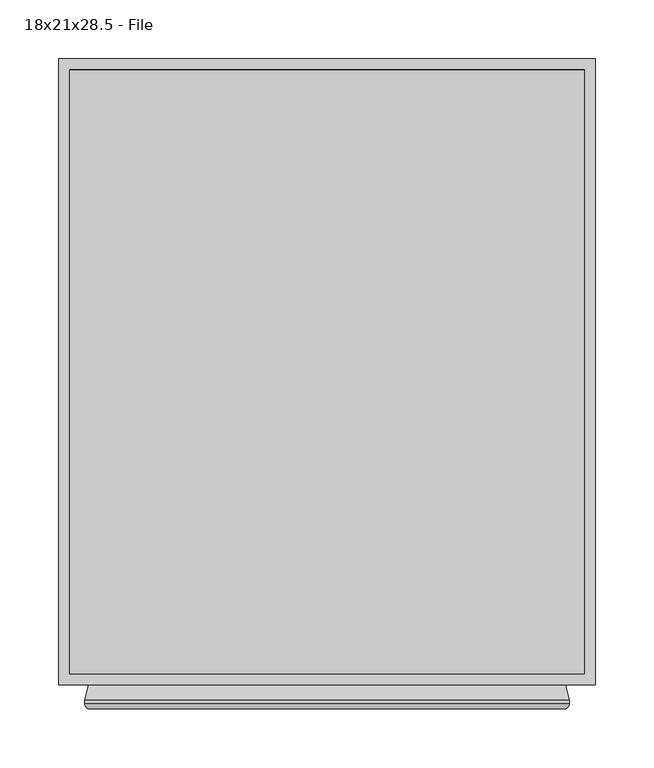
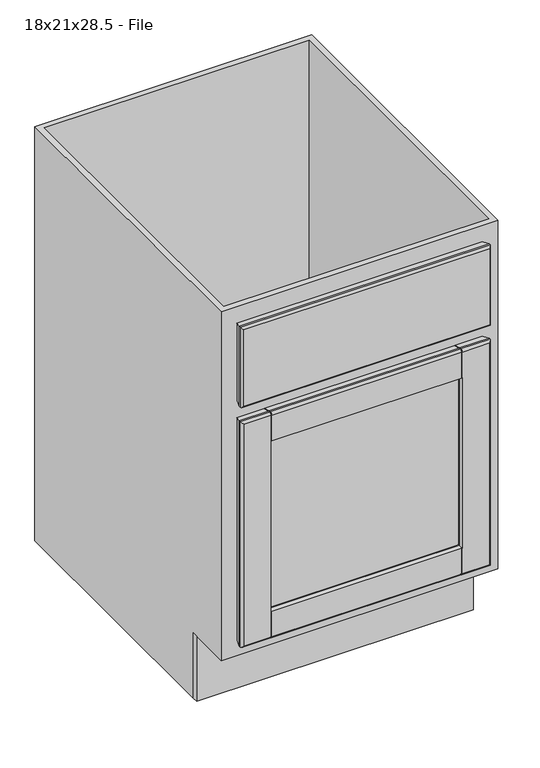
"""IFC4 building model written with IfcOpenShell, lengths in millimetres: furniture geometry, Cabinet-Base-Merillat-Single_Door-Marlin : 18x21x28.5 - File."""

from ifc_helpers import new_model, si_unit, frame, origin, origin_with_axes, place, context, project, spatial, polyline, circle_curve, ellipse_curve, outline, extrude, faceted_brep, source, transform, mapped, element, save
from ifc_brep_helpers import plane_surface, cylinder_surface, advanced_brep


def furniture_18x21x28_5_file_078d9ba0(model_context):
    return source(origin(), model_context, "Body", "SolidModel", [
        advanced_brep(
        [(225.1127049, -625.4496, 533.4), (222.0162124, -629.92, 530.3035075), (222.0162124, -629.92, 142.7964925), (225.1127049, -625.4496, 139.7), (225.1127049, -622.681, 139.7), (225.1127049, -622.681, 533.4), (221.6075049, -609.6, 143.2052), (221.6075049, -609.6, 529.8948), (176.9115422, -609.6, 485.1988372), (176.9115422, -609.6, 187.9011628), (176.5414105, -610.39375, 188.2712945), (174.4602514, -614.85681, 190.3524535), (174.4602514, -614.85681, 482.7475465), (176.5414105, -610.39375, 484.8287055), (175.8600209, -617.0969093, 188.952684), (175.8600209, -617.0969093, 484.147316), (190.1877049, -617.347, 174.625), (190.1877049, -617.347, 498.475), (190.1877049, -622.173, 174.625), (190.1877049, -622.173, 498.475), (175.8600209, -622.4230907, 188.952684), (175.8600209, -622.4230907, 484.147316), (174.4602514, -624.66319, 190.3524535), (174.4602514, -624.66319, 482.7475465), (176.5414105, -629.12625, 188.2712945), (176.9086747, -629.9138508, 187.9040302), (176.9115422, -629.92, 485.1988372), (176.5414105, -629.12625, 484.8287055), (176.9086747, -629.92, 142.7964925), (176.9086747, -625.4496, 139.7), (-184.5408026, -629.92, 142.7964925), (-187.6372951, -625.4496, 139.7), (-139.4730764, -625.4496, 139.7), (-139.4730764, -629.92, 142.7964925), (175.3211747, -625.4496, 139.7), (175.3211747, -629.92, 142.7964925), (-137.8855764, -629.92, 142.7964925), (-137.8855764, -625.4496, 139.7), (176.9086747, -622.681, 139.7), (-187.6372951, -622.681, 139.7), (-139.4730764, -622.681, 139.7), (175.3211747, -622.681, 139.7), (-137.8855764, -622.681, 139.7), (176.9086747, -609.6, 143.2052), (-184.1320951, -609.6, 143.2052), (-139.4730764, -609.6, 143.2052), (175.3211747, -609.6, 143.2052), (-137.8855764, -609.6, 143.2052), (-136.9848416, -614.85681, 190.3524535), (175.3211747, -610.39375, 188.2712945), (175.3211747, -609.6, 187.9011628), (-137.8855764, -609.6, 187.9011628), (-137.8855764, -610.39375, 188.2712945), (-139.0660006, -610.39375, 188.2712945), (-138.384611, -617.0969093, 188.952684), (-152.7122951, -617.347, 174.625), (-152.7122951, -622.173, 174.625), (-138.384611, -622.4230907, 188.952684), (-136.9848416, -624.66319, 190.3524535), (-139.0660006, -629.12625, 188.2712945), (-137.8855764, -629.12625, 188.2712945), (-137.8855764, -629.92, 187.9011628), (175.3211747, -629.92, 187.9011628), (175.3211747, -629.12625, 188.2712945), (-184.5408026, -629.92, 530.3035075), (-187.6372951, -625.4496, 533.4), (-187.6372951, -622.681, 533.4), (-184.1320951, -609.6, 529.8948), (-139.4361323, -609.6, 187.9011628), (-139.4361323, -609.6, 485.1988372), (-139.0660006, -610.39375, 484.8287055), (-136.9848416, -614.85681, 482.7475465), (-138.384611, -617.0969093, 484.147316), (-152.7122951, -617.347, 498.475), (-152.7122951, -622.173, 498.475), (-138.384611, -622.4230907, 484.147316), (-136.9848416, -624.66319, 482.7475465), (-139.0660006, -629.12625, 484.8287055), (-139.4361323, -629.92, 485.1988372), (-139.4361323, -629.92, 187.9011628), (-139.4730764, -629.92, 530.3035075), (-139.4730764, -625.4496, 533.4), (176.9086747, -625.4496, 533.4), (176.9086747, -629.92, 530.3035075), (-137.8855764, -625.4496, 533.4), (-137.8855764, -629.92, 530.3035075), (175.3211747, -629.92, 530.3035075), (175.3211747, -625.4496, 533.4), (-139.4730764, -622.681, 533.4), (176.9086747, -622.681, 533.4), (-137.8855764, -622.681, 533.4), (175.3211747, -622.681, 533.4), (-139.4730764, -609.6, 529.8948), (176.9086747, -609.6, 529.8948), (-137.8855764, -609.6, 529.8948), (175.3211747, -609.6, 529.8948), (-137.8855764, -609.6, 485.1988372), (175.3211747, -609.6, 485.1988372), (-137.8855764, -610.39375, 484.8287055), (175.3211747, -610.39375, 484.8287055), (175.3211747, -629.12625, 484.8287055), (175.3211747, -629.92, 485.1988372), (-137.8855764, -629.92, 485.1988372), (-137.8855764, -629.12625, 484.8287055), (-137.8855764, -610.39375, 529.2857412), (-137.8855764, -622.7855037, 532.60625), (-137.8855764, -625.4496, 532.60625), (-137.8855764, -629.12625, 530.1526052), (-139.4730764, -629.12625, 484.8287055), (-139.4730764, -629.12625, 530.1526052), (-139.4730764, -625.4496, 532.60625), (-139.4730764, -622.7855037, 532.60625), (-139.4730764, -610.39375, 529.2857412), (-139.4730764, -610.39375, 484.8287055), (176.9086747, -610.39375, 484.8287055), (176.9086747, -610.39375, 529.2857412), (176.9086747, -622.7855037, 532.60625), (176.9086747, -625.4496, 532.60625), (176.9086747, -629.12625, 530.1526052), (176.9086747, -629.12625, 484.8287055), (175.3211747, -629.12625, 530.1526052), (175.3211747, -625.4496, 532.60625), (175.3211747, -622.7855037, 532.60625), (175.3211747, -610.39375, 529.2857412), (176.9086747, -629.12625, 188.2712945), (176.9086747, -629.12625, 142.9473948), (176.9086747, -625.4496, 140.49375), (176.9086747, -622.7855037, 140.49375), (176.9086747, -610.39375, 143.8142588), (176.9086747, -610.39375, 188.2712945), (175.3211747, -610.39375, 143.8142588), (175.3211747, -622.7855037, 140.49375), (175.3211747, -625.4496, 140.49375), (175.3211747, -629.12625, 142.9473948), (-137.8855764, -629.12625, 142.9473948), (-137.8855764, -625.4496, 140.49375), (-137.8855764, -622.7855037, 140.49375), (-137.8855764, -610.39375, 143.8142588), (-139.4730764, -629.12625, 188.2712945), (-139.4730764, -610.39375, 188.2712945), (-139.4730764, -610.39375, 143.8142588), (-139.4730764, -622.7855037, 140.49375), (-139.4730764, -625.4496, 140.49375), (-139.4730764, -629.12625, 142.9473948)],
        [
            (0, 1, ellipse_curve(frame((220.3375049, -625.4496, 528.6248), z_axis=(0.7071067811865475, 0.0, -0.7071067811865475), x_axis=(0.7071067811865474, 0.0, 0.7071067811865476)), 6.7531526, 4.7752)),
            (1, 2),
            (2, 3, ellipse_curve(frame((220.3375049, -625.4496, 144.4752), z_axis=(0.7071067811865475, 0.0, 0.7071067811865475), x_axis=(-0.7071067811865474, 0.0, 0.7071067811865476)), 6.7531526, 4.7752)),
            (3, 0),
            (3, 4),
            (4, 5),
            (5, 0),
            (4, 6),
            (6, 7),
            (7, 5),
            (8, 9),
            (9, 10),
            (10, 11),
            (11, 12),
            (12, 13),
            (13, 8),
            (11, 14, ellipse_curve(frame((175.8875049, -615.5223492, 188.9252), z_axis=(0.7071067811865475, 0.0, 0.7071067811865475), x_axis=(-0.7071067811865474, 0.0, 0.7071067811865476)), 2.2271035, 1.5748)),
            (14, 15),
            (15, 12, ellipse_curve(frame((175.8875049, -615.5223492, 484.1748), z_axis=(0.7071067811865475, 0.0, -0.7071067811865475), x_axis=(0.7071067811865474, 0.0, 0.7071067811865476)), 2.2271035, 1.5748)),
            (14, 16),
            (16, 17),
            (17, 15),
            (16, 18),
            (18, 19),
            (19, 17),
            (18, 20),
            (20, 21),
            (21, 19),
            (20, 22, ellipse_curve(frame((175.8875049, -623.9976508, 188.9252), z_axis=(0.7071067811865475, 0.0, 0.7071067811865475), x_axis=(-0.7071067811865474, 0.0, 0.7071067811865476)), 2.2271035, 1.5748)),
            (22, 23),
            (23, 21, ellipse_curve(frame((175.8875049, -623.9976508, 484.1748), z_axis=(0.7071067811865475, 0.0, -0.7071067811865475), x_axis=(0.7071067811865474, 0.0, 0.7071067811865476)), 2.2271035, 1.5748)),
            (22, 24),
            (24, 25),
            (25, 26),
            (26, 27),
            (27, 23),
            (2, 28),
            (28, 29, circle_curve(frame((176.9086747, -625.4496, 144.4752), z_axis=(1.0, 0.0, 0.0), x_axis=(0.0, 1.0, 0.0)), 4.7752)),
            (29, 3),
            (30, 31, ellipse_curve(frame((-182.8620951, -625.4496, 144.4752), z_axis=(0.7071067811865475, 0.0, -0.7071067811865475), x_axis=(0.7071067811865476, 0.0, 0.7071067811865474)), 6.7531526, 4.7752)),
            (31, 32),
            (32, 33, circle_curve(frame((-139.4730764, -625.4496, 144.4752), z_axis=(-1.0, 0.0, 0.0), x_axis=(0.0, 1.0, 0.0)), 4.7752)),
            (33, 30),
            (34, 35, circle_curve(frame((175.3211747, -625.4496, 144.4752), z_axis=(-1.0, 0.0, 0.0), x_axis=(0.0, 1.0, 0.0)), 4.7752)),
            (35, 36),
            (36, 37, circle_curve(frame((-137.8855764, -625.4496, 144.4752), z_axis=(1.0, 0.0, 0.0), x_axis=(0.0, 1.0, 0.0)), 4.7752)),
            (37, 34),
            (29, 38),
            (38, 4),
            (31, 39),
            (39, 40),
            (40, 32),
            (41, 34),
            (37, 42),
            (42, 41),
            (38, 43),
            (43, 6),
            (39, 44),
            (44, 45),
            (45, 40),
            (46, 41),
            (42, 47),
            (47, 46),
            (48, 11),
            (10, 49),
            (49, 50),
            (50, 51),
            (51, 52),
            (52, 53),
            (53, 48),
            (48, 54, ellipse_curve(frame((-138.4120951, -615.5223492, 188.9252), z_axis=(0.7071067811865475, 0.0, -0.7071067811865475), x_axis=(0.7071067811865476, 0.0, 0.7071067811865474)), 2.2271035, 1.5748)),
            (54, 14),
            (54, 55),
            (55, 16),
            (55, 56),
            (56, 18),
            (56, 57),
            (57, 20),
            (57, 58, ellipse_curve(frame((-138.4120951, -623.9976508, 188.9252), z_axis=(0.7071067811865475, 0.0, -0.7071067811865475), x_axis=(0.7071067811865476, 0.0, 0.7071067811865474)), 2.2271035, 1.5748)),
            (58, 22),
            (58, 59),
            (59, 60),
            (60, 61),
            (61, 62),
            (62, 63),
            (63, 24),
            (30, 64),
            (64, 65, ellipse_curve(frame((-182.8620951, -625.4496, 528.6248), z_axis=(-0.7071067811865475, 0.0, -0.7071067811865475), x_axis=(0.7071067811865474, 0.0, -0.7071067811865476)), 6.7531526, 4.7752)),
            (65, 31),
            (65, 66),
            (66, 39),
            (66, 67),
            (67, 44),
            (68, 69),
            (69, 70),
            (70, 71),
            (71, 48),
            (53, 68),
            (71, 72, ellipse_curve(frame((-138.4120951, -615.5223492, 484.1748), z_axis=(-0.7071067811865475, 0.0, -0.7071067811865475), x_axis=(0.7071067811865474, 0.0, -0.7071067811865476)), 2.2271035, 1.5748)),
            (72, 54),
            (72, 73),
            (73, 55),
            (73, 74),
            (74, 56),
            (74, 75),
            (75, 57),
            (75, 76, ellipse_curve(frame((-138.4120951, -623.9976508, 484.1748), z_axis=(-0.7071067811865475, 0.0, -0.7071067811865475), x_axis=(0.7071067811865474, 0.0, -0.7071067811865476)), 2.2271035, 1.5748)),
            (76, 58),
            (76, 77),
            (77, 78),
            (78, 79),
            (79, 59),
            (64, 80),
            (80, 81, circle_curve(frame((-139.4730764, -625.4496, 528.6248), z_axis=(-1.0, 0.0, 0.0), x_axis=(0.0, 1.0, 0.0)), 4.7752)),
            (81, 65),
            (0, 82),
            (82, 83, circle_curve(frame((176.9086747, -625.4496, 528.6248), z_axis=(1.0, 0.0, 0.0), x_axis=(0.0, 1.0, 0.0)), 4.7752)),
            (83, 1),
            (84, 85, circle_curve(frame((-137.8855764, -625.4496, 528.6248), z_axis=(1.0, 0.0, 0.0), x_axis=(0.0, 1.0, 0.0)), 4.7752)),
            (85, 86),
            (86, 87, circle_curve(frame((175.3211747, -625.4496, 528.6248), z_axis=(-1.0, 0.0, 0.0), x_axis=(0.0, 1.0, 0.0)), 4.7752)),
            (87, 84),
            (81, 88),
            (88, 66),
            (5, 89),
            (89, 82),
            (90, 84),
            (87, 91),
            (91, 90),
            (88, 92),
            (92, 67),
            (7, 93),
            (93, 89),
            (94, 90),
            (91, 95),
            (95, 94),
            (43, 9),
            (8, 93),
            (92, 69),
            (68, 45),
            (96, 94),
            (95, 97),
            (97, 96),
            (50, 46),
            (47, 51),
            (12, 71),
            (70, 98),
            (98, 96),
            (97, 99),
            (99, 13),
            (15, 72),
            (17, 73),
            (19, 74),
            (21, 75),
            (23, 76),
            (27, 100),
            (100, 101),
            (101, 102),
            (102, 103),
            (103, 77),
            (83, 26),
            (25, 28),
            (33, 79),
            (78, 80),
            (85, 102),
            (101, 86),
            (35, 62),
            (61, 36),
            (98, 104),
            (104, 105),
            (105, 106),
            (106, 107, circle_curve(frame((-137.8855764, -625.4496, 528.6248), z_axis=(1.0, 0.0, 0.0), x_axis=(0.0, 0.0, 1.0)), 3.98145)),
            (107, 103),
            (78, 108),
            (108, 109),
            (109, 110, circle_curve(frame((-139.4730764, -625.4496, 528.6248), z_axis=(-1.0, 0.0, 0.0), x_axis=(0.0, 0.0, 1.0)), 3.98145)),
            (110, 111),
            (111, 112),
            (112, 113),
            (113, 69),
            (77, 108),
            (107, 109),
            (106, 110),
            (105, 111),
            (104, 112),
            (70, 113),
            (8, 114),
            (114, 115),
            (115, 116),
            (116, 117),
            (117, 118, circle_curve(frame((176.9086747, -625.4496, 528.6248), z_axis=(1.0, 0.0, 0.0), x_axis=(0.0, 0.0, 1.0)), 3.98145)),
            (118, 119),
            (119, 26),
            (100, 120),
            (120, 121, circle_curve(frame((175.3211747, -625.4496, 528.6248), z_axis=(-1.0, 0.0, 0.0), x_axis=(0.0, 0.0, 1.0)), 3.98145)),
            (121, 122),
            (122, 123),
            (123, 99),
            (119, 27),
            (118, 120),
            (117, 121),
            (116, 122),
            (115, 123),
            (114, 13),
            (25, 124),
            (124, 125),
            (125, 126, circle_curve(frame((176.9086747, -625.4496, 144.4752), z_axis=(1.0, 0.0, 0.0), x_axis=(0.0, 0.0, 1.0)), 3.98145)),
            (126, 127),
            (127, 128),
            (128, 129),
            (129, 9),
            (49, 130),
            (130, 131),
            (131, 132),
            (132, 133, circle_curve(frame((175.3211747, -625.4496, 144.4752), z_axis=(-1.0, 0.0, 0.0), x_axis=(0.0, 0.0, 1.0)), 3.98145)),
            (133, 63),
            (129, 10),
            (128, 130),
            (127, 131),
            (126, 132),
            (125, 133),
            (124, 24),
            (60, 134),
            (134, 135, circle_curve(frame((-137.8855764, -625.4496, 144.4752), z_axis=(1.0, 0.0, 0.0), x_axis=(0.0, 0.0, 1.0)), 3.98145)),
            (135, 136),
            (136, 137),
            (137, 52),
            (138, 79),
            (68, 139),
            (139, 140),
            (140, 141),
            (141, 142),
            (142, 143, circle_curve(frame((-139.4730764, -625.4496, 144.4752), z_axis=(-1.0, 0.0, 0.0), x_axis=(0.0, 0.0, 1.0)), 3.98145)),
            (143, 138),
            (138, 59),
            (53, 139),
            (137, 140),
            (136, 141),
            (135, 142),
            (134, 143),
        ],
        [
            cylinder_surface(frame((220.3375049, -625.4496, 533.4), z_axis=(0.0, 0.0, 1.0), x_axis=(0.0, 1.0, 0.0)), 4.7752),
            plane_surface(frame((225.1127049, -625.4496, 533.4), z_axis=(1.0, 0.0, 0.0), x_axis=(0.0, 0.0, -1.0))),
            plane_surface(frame((225.1127049, -622.681, 533.4), z_axis=(0.9659229350723619, 0.25882983502910506, 0.0), x_axis=(0.0, 0.0, -1.0))),
            plane_surface(frame((176.9115422, -609.6, 485.1988372), z_axis=(-0.9063077870366099, 0.4226182617407856, 0.0), x_axis=(0.0, 0.0, -1.0))),
            cylinder_surface(frame((175.8875049, -615.5223492, 533.4), z_axis=(0.0, 0.0, 1.0000000000000002), x_axis=(-0.01745240643729364, -0.9998476951563912, 0.0)), 1.5748),
            plane_surface(frame((175.8600209, -617.0969093, 484.147316), z_axis=(-0.017452406437322144, -0.9998476951563906, 0.0), x_axis=(0.0, 0.0, -1.0))),
            plane_surface(frame((190.1877049, -617.347, 498.475), z_axis=(-1.0, 0.0, 0.0), x_axis=(0.0, 0.0, -1.0))),
            plane_surface(frame((190.1877049, -622.173, 498.475), z_axis=(-0.01745240643727848, 0.9998476951563914, 0.0), x_axis=(0.0, 0.0, -1.0))),
            cylinder_surface(frame((175.8875049, -623.9976508, 533.4), z_axis=(0.0, 0.0, 1.0000000000000002), x_axis=(-0.9063077870367326, -0.42261826174052236, 0.0)), 1.5748),
            plane_surface(frame((174.4602514, -624.66319, 482.7475465), z_axis=(-0.9063077870366333, -0.4226182617407352, 0.0), x_axis=(0.0, 0.0, -1.0))),
            cylinder_surface(frame((225.1127049, -625.4496, 144.4752), z_axis=(1.0, 0.0, 0.0), x_axis=(0.0, 1.0, 0.0)), 4.7752),
            plane_surface(frame((225.1127049, -625.4496, 139.7), z_axis=(0.0, 0.0, -1.0), x_axis=(-1.0, 0.0, 0.0))),
            plane_surface(frame((225.1127049, -622.681, 139.7), z_axis=(0.0, 0.25882983502910506, -0.9659229350723619), x_axis=(-1.0, 0.0, 0.0))),
            plane_surface(frame((176.9115422, -609.6, 187.9011628), z_axis=(0.0, 0.4226182617407856, 0.9063077870366099), x_axis=(-1.0, 0.0, 0.0))),
            cylinder_surface(frame((225.1127049, -615.5223492, 188.9252), z_axis=(1.0000000000000002, 0.0, 0.0), x_axis=(0.0, -0.9998476951563912, 0.01745240643729364)), 1.5748),
            plane_surface(frame((175.8600209, -617.0969093, 188.952684), z_axis=(0.0, -0.9998476951563906, 0.017452406437322144), x_axis=(-1.0, 0.0, 0.0))),
            plane_surface(frame((190.1877049, -617.347, 174.625), z_axis=(0.0, 0.0, 1.0), x_axis=(-1.0, 0.0, 0.0))),
            plane_surface(frame((190.1877049, -622.173, 174.625), z_axis=(0.0, 0.9998476951563914, 0.01745240643727848), x_axis=(-1.0, 0.0, 0.0))),
            cylinder_surface(frame((225.1127049, -623.9976508, 188.9252), z_axis=(1.0000000000000002, 0.0, 0.0), x_axis=(0.0, -0.42261826174052236, 0.9063077870367326)), 1.5748),
            plane_surface(frame((174.4602514, -624.66319, 190.3524535), z_axis=(0.0, -0.4226182617407352, 0.9063077870366333), x_axis=(-1.0, 0.0, 0.0))),
            cylinder_surface(frame((-182.8620951, -625.4496, 139.7), z_axis=(0.0, 0.0, -1.0), x_axis=(0.0, 1.0, 0.0)), 4.7752),
            plane_surface(frame((-187.6372951, -625.4496, 139.7), z_axis=(-1.0, 0.0, 0.0), x_axis=(0.0, 0.0, 1.0))),
            plane_surface(frame((-187.6372951, -622.681, 139.7), z_axis=(-0.9659229350723619, 0.25882983502910506, 0.0), x_axis=(0.0, 0.0, 1.0))),
            plane_surface(frame((-139.4361323, -609.6, 187.9011628), z_axis=(0.9063077870366099, 0.4226182617407856, 0.0), x_axis=(0.0, 0.0, 1.0))),
            cylinder_surface(frame((-138.4120951, -615.5223492, 139.7), z_axis=(0.0, 0.0, -1.0000000000000002), x_axis=(0.01745240643729364, -0.9998476951563912, 0.0)), 1.5748),
            plane_surface(frame((-138.384611, -617.0969093, 188.952684), z_axis=(0.017452406437322144, -0.9998476951563906, 0.0), x_axis=(0.0, 0.0, 1.0))),
            plane_surface(frame((-152.7122951, -617.347, 174.625), z_axis=(1.0, 0.0, 0.0), x_axis=(0.0, 0.0, 1.0))),
            plane_surface(frame((-152.7122951, -622.173, 174.625), z_axis=(0.01745240643727848, 0.9998476951563914, 0.0), x_axis=(0.0, 0.0, 1.0))),
            cylinder_surface(frame((-138.4120951, -623.9976508, 139.7), z_axis=(0.0, 0.0, -1.0000000000000002), x_axis=(0.9063077870367326, -0.42261826174052236, 0.0)), 1.5748),
            plane_surface(frame((-136.9848416, -624.66319, 190.3524535), z_axis=(0.9063077870366333, -0.4226182617407352, 0.0), x_axis=(0.0, 0.0, 1.0))),
            cylinder_surface(frame((-187.6372951, -625.4496, 528.6248), z_axis=(-1.0, 0.0, 0.0), x_axis=(0.0, 1.0, 0.0)), 4.7752),
            plane_surface(frame((-187.6372951, -625.4496, 533.4), z_axis=(0.0, 0.0, 1.0), x_axis=(1.0, 0.0, 0.0))),
            plane_surface(frame((-187.6372951, -622.681, 533.4), z_axis=(0.0, 0.25882983502910506, 0.9659229350723619), x_axis=(1.0, 0.0, 0.0))),
            plane_surface(frame((-184.1320951, -609.6, 529.8948), z_axis=(0.0, 1.0, 0.0), x_axis=(1.0, 0.0, 0.0))),
            plane_surface(frame((-139.4361323, -609.6, 485.1988372), z_axis=(0.0, 0.4226182617407856, -0.9063077870366099), x_axis=(1.0, 0.0, 0.0))),
            cylinder_surface(frame((-187.6372951, -615.5223492, 484.1748), z_axis=(-1.0000000000000002, 0.0, 0.0), x_axis=(0.0, -0.9998476951563912, -0.01745240643729364)), 1.5748),
            plane_surface(frame((-138.384611, -617.0969093, 484.147316), z_axis=(0.0, -0.9998476951563906, -0.017452406437322144), x_axis=(1.0, 0.0, 0.0))),
            plane_surface(frame((-152.7122951, -617.347, 498.475), z_axis=(0.0, 0.0, -1.0), x_axis=(1.0, 0.0, 0.0))),
            plane_surface(frame((-152.7122951, -622.173, 498.475), z_axis=(0.0, 0.9998476951563914, -0.01745240643727848), x_axis=(1.0, 0.0, 0.0))),
            cylinder_surface(frame((-187.6372951, -623.9976508, 484.1748), z_axis=(-1.0000000000000002, 0.0, 0.0), x_axis=(0.0, -0.42261826174052236, -0.9063077870367326)), 1.5748),
            plane_surface(frame((-136.9848416, -624.66319, 482.7475465), z_axis=(0.0, -0.4226182617407352, -0.9063077870366333), x_axis=(1.0, 0.0, 0.0))),
            plane_surface(frame((-139.4361323, -629.92, 485.1988372), z_axis=(0.0, -1.0, 0.0), x_axis=(1.0, 0.0, 0.0))),
            plane_surface(frame((-137.8855764, -629.92, 485.1988372), z_axis=(-1.0000000000000002, 0.0, 0.0), x_axis=(0.0, 0.9063077870366303, -0.4226182617407418))),
            plane_surface(frame((-139.4730764, -629.92, 485.1988372), z_axis=(1.0000000000000002, 0.0, 0.0), x_axis=(0.0, -0.9063077870366303, 0.4226182617407418))),
            plane_surface(frame((-137.8855764, -629.92, 485.1988372), z_axis=(0.0, 0.4226182617407418, 0.9063077870366303), x_axis=(-1.0, 0.0, 0.0))),
            plane_surface(frame((-137.8855764, -629.12625, 484.8287055), z_axis=(0.0, -1.0, 0.0), x_axis=(-1.0, 0.0, 0.0))),
            cylinder_surface(frame((-139.4730764, -625.4496, 528.6248), z_axis=(-1.0, 0.0, 0.0), x_axis=(0.0, 0.0, 1.0)), 3.98145),
            plane_surface(frame((-137.8855764, -625.4496, 532.60625), z_axis=(0.0, 0.0, 1.0), x_axis=(-1.0, 0.0, 0.0))),
            plane_surface(frame((-137.8855764, -622.7855037, 532.60625), z_axis=(0.0, 0.25882983502916795, 0.9659229350723451), x_axis=(-1.0, 0.0, 0.0))),
            plane_surface(frame((-137.8855764, -610.39375, 529.2857412), z_axis=(0.0, 1.0, 0.0), x_axis=(-1.0, 0.0, 0.0))),
            plane_surface(frame((-137.8855764, -610.39375, 484.8287055), z_axis=(0.0, -0.4226182617407951, 0.9063077870366054), x_axis=(-1.0, 0.0, 0.0))),
            plane_surface(frame((176.9086747, -629.92, 485.1988372), z_axis=(-1.0, 0.0, 0.0), x_axis=(0.0, 0.9063077870366284, -0.42261826174074574))),
            plane_surface(frame((175.3211747, -629.92, 485.1988372), z_axis=(1.0, 0.0, 0.0), x_axis=(0.0, -0.9063077870366284, 0.42261826174074574))),
            plane_surface(frame((176.9086747, -629.92, 485.1988372), z_axis=(0.0, 0.42261826174074574, 0.9063077870366284), x_axis=(-1.0, 0.0, 0.0))),
            plane_surface(frame((176.9086747, -629.12625, 484.8287055), z_axis=(0.0, -1.0, 0.0), x_axis=(-1.0, 0.0, 0.0))),
            cylinder_surface(frame((175.3211747, -625.4496, 528.6248), z_axis=(-1.0, 0.0, 0.0), x_axis=(0.0, 0.0, 1.0)), 3.98145),
            plane_surface(frame((176.9086747, -625.4496, 532.60625), z_axis=(0.0, 0.0, 1.0), x_axis=(-1.0, 0.0, 0.0))),
            plane_surface(frame((176.9086747, -622.7855037, 532.60625), z_axis=(0.0, 0.25882983502917023, 0.9659229350723445), x_axis=(-1.0, 0.0, 0.0))),
            plane_surface(frame((176.9086747, -610.39375, 529.2857412), z_axis=(0.0, 1.0, 0.0), x_axis=(-1.0, 0.0, 0.0))),
            plane_surface(frame((176.9086747, -610.39375, 484.8287055), z_axis=(0.0, -0.4226182617408056, 0.9063077870366005), x_axis=(-1.0, 0.0, 0.0))),
            plane_surface(frame((176.9086747, -625.4496, 149.2504), z_axis=(-1.0, 0.0, 0.0), x_axis=(0.0, -1.0, 0.0))),
            plane_surface(frame((175.3211747, -625.4496, 149.2504), z_axis=(1.0, 0.0, 0.0), x_axis=(0.0, 1.0, 0.0))),
            plane_surface(frame((176.9086747, -609.6, 187.9011628), z_axis=(0.0, -0.4226182617407918, -0.906307787036607), x_axis=(-1.0, 0.0, 0.0))),
            plane_surface(frame((176.9086747, -610.39375, 188.2712945), z_axis=(0.0, 1.0, 0.0), x_axis=(-1.0, 0.0, 0.0))),
            plane_surface(frame((176.9086747, -610.39375, 143.8142588), z_axis=(0.0, 0.25882983502943885, -0.9659229350722724), x_axis=(-1.0, 0.0, 0.0))),
            plane_surface(frame((176.9086747, -622.7855037, 140.49375), z_axis=(0.0, 0.0, -1.0), x_axis=(-1.0, 0.0, 0.0))),
            cylinder_surface(frame((175.3211747, -625.4496, 144.4752), z_axis=(-1.0, 0.0, 0.0), x_axis=(0.0, 0.0, 1.0)), 3.98145),
            plane_surface(frame((176.9086747, -629.12625, 142.9473948), z_axis=(0.0, -1.0, 0.0), x_axis=(-1.0, 0.0, 0.0))),
            plane_surface(frame((176.9086747, -629.12625, 188.2712945), z_axis=(0.0, 0.42261826174073464, -0.9063077870366336), x_axis=(-1.0, 0.0, 0.0))),
            plane_surface(frame((-137.8855764, -629.12625, 188.2712945), z_axis=(-1.0, 0.0, 0.0), x_axis=(0.0, -0.9063077870366311, -0.4226182617407399))),
            plane_surface(frame((-139.4730764, -629.12625, 188.2712945), z_axis=(1.0, 0.0, 0.0), x_axis=(0.0, 0.9063077870366311, 0.4226182617407399))),
            plane_surface(frame((-137.8855764, -629.12625, 188.2712945), z_axis=(0.0, 0.4226182617407399, -0.9063077870366311), x_axis=(-1.0, 0.0, 0.0))),
            plane_surface(frame((-137.8855764, -609.6, 187.9011628), z_axis=(0.0, -0.42261826174079353, -0.9063077870366061), x_axis=(-1.0, 0.0, 0.0))),
            plane_surface(frame((-137.8855764, -610.39375, 188.2712945), z_axis=(0.0, 1.0, 0.0), x_axis=(-1.0, 0.0, 0.0))),
            plane_surface(frame((-137.8855764, -610.39375, 143.8142588), z_axis=(0.0, 0.2588298350294384, -0.9659229350722726), x_axis=(-1.0, 0.0, 0.0))),
            plane_surface(frame((-137.8855764, -622.7855037, 140.49375), z_axis=(0.0, 0.0, -1.0), x_axis=(-1.0, 0.0, 0.0))),
            cylinder_surface(frame((-139.4730764, -625.4496, 144.4752), z_axis=(-1.0, 0.0, 0.0), x_axis=(0.0, 0.0, 1.0)), 3.98145),
            plane_surface(frame((-137.8855764, -629.12625, 142.9473948), z_axis=(0.0, -1.0, 0.0), x_axis=(-1.0, 0.0, 0.0))),
        ],
        [
            (0, [[1, 2, 3, 4]]),
            (1, [[-4, 5, 6, 7]]),
            (2, [[-6, 8, 9, 10]]),
            (3, [[11, 12, 13, 14, 15, 16]]),
            (4, [[-14, 17, 18, 19]]),
            (5, [[-18, 20, 21, 22]]),
            (6, [[-21, 23, 24, 25]]),
            (7, [[-24, 26, 27, 28]]),
            (8, [[-27, 29, 30, 31]]),
            (9, [[-30, 32, 33, 34, 35, 36]]),
            (10, [[-3, 37, 38, 39]]),
            (10, [[40, 41, 42, 43]]),
            (10, [[44, 45, 46, 47]]),
            (11, [[-5, -39, 48, 49]]),
            (11, [[50, 51, 52, -41]]),
            (11, [[53, -47, 54, 55]]),
            (12, [[-8, -49, 56, 57]]),
            (12, [[58, 59, 60, -51]]),
            (12, [[61, -55, 62, 63]]),
            (13, [[64, -13, 65, 66, 67, 68, 69, 70]]),
            (14, [[-17, -64, 71, 72]]),
            (15, [[-20, -72, 73, 74]]),
            (16, [[-23, -74, 75, 76]]),
            (17, [[-26, -76, 77, 78]]),
            (18, [[-29, -78, 79, 80]]),
            (19, [[-80, 81, 82, 83, 84, 85, 86, -32]]),
            (20, [[-40, 87, 88, 89]]),
            (21, [[-50, -89, 90, 91]]),
            (22, [[-58, -91, 92, 93]]),
            (23, [[94, 95, 96, 97, -70, 98]]),
            (24, [[-71, -97, 99, 100]]),
            (25, [[-73, -100, 101, 102]]),
            (26, [[-75, -102, 103, 104]]),
            (27, [[-77, -104, 105, 106]]),
            (28, [[-79, -106, 107, 108]]),
            (29, [[-108, 109, 110, 111, 112, -81]]),
            (30, [[-88, 113, 114, 115]]),
            (30, [[-1, 116, 117, 118]]),
            (30, [[119, 120, 121, 122]]),
            (31, [[-90, -115, 123, 124]]),
            (31, [[-7, 125, 126, -116]]),
            (31, [[127, -122, 128, 129]]),
            (32, [[-92, -124, 130, 131]]),
            (32, [[-10, 132, 133, -125]]),
            (32, [[134, -129, 135, 136]]),
            (33, [[-9, -57, 137, -11, 138, -132]]),
            (33, [[-93, -131, 139, -94, 140, -59]]),
            (33, [[141, -136, 142, 143]]),
            (33, [[144, -63, 145, -67]]),
            (34, [[146, -96, 147, 148, -143, 149, 150, -15]]),
            (35, [[-19, 151, -99, -146]]),
            (36, [[-22, 152, -101, -151]]),
            (37, [[-25, 153, -103, -152]]),
            (38, [[-28, 154, -105, -153]]),
            (39, [[-31, 155, -107, -154]]),
            (40, [[-155, -36, 156, 157, 158, 159, 160, -109]]),
            (41, [[-2, -118, 161, -34, 162, -37]]),
            (41, [[-87, -43, 163, -111, 164, -113]]),
            (41, [[165, -158, 166, -120]]),
            (41, [[167, -84, 168, -45]]),
            (42, [[169, 170, 171, 172, 173, -159, -165, -119, -127, -134, -141, -148]]),
            (43, [[174, 175, 176, 177, 178, 179, 180, -139, -130, -123, -114, -164]]),
            (44, [[-174, -110, 181]]),
            (45, [[-173, 182, -175, -181, -160]]),
            (46, [[-172, 183, -176, -182]]),
            (47, [[-171, 184, -177, -183]]),
            (48, [[-170, 185, -178, -184]]),
            (49, [[-169, -147, 186, -179, -185]]),
            (50, [[-180, -186, -95]]),
            (51, [[187, 188, 189, 190, 191, 192, 193, -161, -117, -126, -133, -138]]),
            (52, [[194, 195, 196, 197, 198, -149, -142, -135, -128, -121, -166, -157]]),
            (53, [[-193, 199, -35]]),
            (54, [[-192, 200, -194, -156, -199]]),
            (55, [[-191, 201, -195, -200]]),
            (56, [[-190, 202, -196, -201]]),
            (57, [[-189, 203, -197, -202]]),
            (58, [[-188, 204, -150, -198, -203]]),
            (59, [[-187, -16, -204]]),
            (60, [[205, 206, 207, 208, 209, 210, 211, -137, -56, -48, -38, -162]]),
            (61, [[212, 213, 214, 215, 216, -85, -167, -44, -53, -61, -144, -66]]),
            (62, [[-211, 217, -12]]),
            (63, [[-210, 218, -212, -65, -217]]),
            (64, [[-209, 219, -213, -218]]),
            (65, [[-208, 220, -214, -219]]),
            (66, [[-207, 221, -215, -220]]),
            (67, [[-206, 222, -86, -216, -221]]),
            (68, [[-205, -33, -222]]),
            (69, [[223, 224, 225, 226, 227, -68, -145, -62, -54, -46, -168, -83]]),
            (70, [[228, -163, -42, -52, -60, -140, 229, 230, 231, 232, 233, 234]]),
            (71, [[-228, 235, -112]]),
            (72, [[-229, -98, 236]]),
            (73, [[-227, 237, -230, -236, -69]]),
            (74, [[-226, 238, -231, -237]]),
            (75, [[-225, 239, -232, -238]]),
            (76, [[-224, 240, -233, -239]]),
            (77, [[-223, -82, -235, -234, -240]]),
        ],
    ),
        extrude(outline(polyline([(-152.7122951, -622.173), (-152.7122951, -617.347), (190.1877049, -617.347), (190.1877049, -622.173), (-152.7122951, -622.173)])), frame((0.0, 0.0, 174.625), z_axis=(0.0, 0.0, 1.0), x_axis=(1.0, 0.0, 0.0)), (0.0, 0.0, 1.0), 323.85),
        advanced_brep(
        [(-184.5408026, -629.92, 695.4035075), (-184.5408026, -629.92, 561.8964925), (222.0162124, -629.92, 561.8964925), (222.0162124, -629.92, 695.4035075), (-184.1320951, -609.6, 562.3052), (-184.1320951, -609.6, 694.9948), (221.6075049, -609.6, 694.9948), (221.6075049, -609.6, 562.3052), (-187.6372951, -625.4496, 698.5), (-187.6372951, -622.681, 698.5), (-187.6372951, -622.681, 558.8), (-187.6372951, -625.4496, 558.8), (225.1127049, -622.681, 558.8), (225.1127049, -625.4496, 558.8), (225.1127049, -622.681, 698.5), (225.1127049, -625.4496, 698.5)],
        [
            (0, 1),
            (1, 2),
            (2, 3),
            (3, 0),
            (4, 5),
            (5, 6),
            (6, 7),
            (7, 4),
            (8, 9),
            (9, 10),
            (10, 11),
            (11, 8),
            (10, 12),
            (12, 13),
            (13, 11),
            (12, 14),
            (14, 15),
            (15, 13),
            (8, 15),
            (14, 9),
            (11, 1, ellipse_curve(frame((-182.8620951, -625.4496, 563.5752), z_axis=(-0.7071067811865475, 0.0, 0.7071067811865475), x_axis=(-0.7071067811865474, 0.0, -0.7071067811865476)), 6.7531526, 4.7752)),
            (0, 8, ellipse_curve(frame((-182.8620951, -625.4496, 693.7248), z_axis=(-0.7071067811865475, 0.0, -0.7071067811865475), x_axis=(0.7071067811865474, 0.0, -0.7071067811865476)), 6.7531526, 4.7752)),
            (4, 10),
            (9, 5),
            (13, 2, ellipse_curve(frame((220.3375049, -625.4496, 563.5752), z_axis=(-0.7071067811865475, 0.0, -0.7071067811865475), x_axis=(0.7071067811865476, 0.0, -0.7071067811865474)), 6.7531526, 4.7752)),
            (7, 12),
            (15, 3, ellipse_curve(frame((220.3375049, -625.4496, 693.7248), z_axis=(0.7071067811865475, 0.0, -0.7071067811865475), x_axis=(0.7071067811865474, 0.0, 0.7071067811865476)), 6.7531526, 4.7752)),
            (6, 14),
        ],
        [
            plane_surface(frame((-187.6372951, -629.92, 698.5), z_axis=(0.0, -1.0, 0.0), x_axis=(0.0, 0.0, -1.0))),
            plane_surface(frame((-187.6372951, -609.6, 698.5), z_axis=(0.0, 1.0, 0.0), x_axis=(0.0, 0.0, 1.0))),
            plane_surface(frame((-187.6372951, -629.92, 698.5), z_axis=(-1.0, 0.0, 0.0), x_axis=(0.0, 1.0, 0.0))),
            plane_surface(frame((-187.6372951, -629.92, 558.8), z_axis=(0.0, 0.0, -1.0), x_axis=(0.0, 1.0, 0.0))),
            plane_surface(frame((225.1127049, -629.92, 558.8), z_axis=(1.0, 0.0, 0.0), x_axis=(0.0, 1.0, 0.0))),
            plane_surface(frame((225.1127049, -629.92, 698.5), z_axis=(0.0, 0.0, 1.0), x_axis=(0.0, 1.0, 0.0))),
            cylinder_surface(frame((-182.8620951, -625.4496, 698.5), z_axis=(0.0, 0.0, -1.0), x_axis=(0.0, 1.0, 0.0)), 4.7752),
            plane_surface(frame((-187.6372951, -622.681, 698.5), z_axis=(-0.9659229350723619, 0.25882983502910506, 0.0), x_axis=(0.0, 0.0, -1.0))),
            cylinder_surface(frame((-187.6372951, -625.4496, 563.5752), z_axis=(1.0, 0.0, 0.0), x_axis=(0.0, 1.0, 0.0)), 4.7752),
            plane_surface(frame((-187.6372951, -622.681, 558.8), z_axis=(0.0, 0.25882983502910506, -0.9659229350723619), x_axis=(1.0, 0.0, 0.0))),
            cylinder_surface(frame((220.3375049, -625.4496, 558.8), z_axis=(0.0, 0.0, 1.0), x_axis=(0.0, 1.0, 0.0)), 4.7752),
            plane_surface(frame((225.1127049, -622.681, 558.8), z_axis=(0.9659229350723619, 0.25882983502910506, 0.0), x_axis=(0.0, 0.0, 1.0))),
            cylinder_surface(frame((225.1127049, -625.4496, 693.7248), z_axis=(-1.0, 0.0, 0.0), x_axis=(0.0, 1.0, 0.0)), 4.7752),
            plane_surface(frame((225.1127049, -622.681, 698.5), z_axis=(0.0, 0.25882983502910506, 0.9659229350723619), x_axis=(-1.0, 0.0, 0.0))),
        ],
        [
            (0, [[1, 2, 3, 4]]),
            (1, [[5, 6, 7, 8]]),
            (2, [[9, 10, 11, 12]]),
            (3, [[-11, 13, 14, 15]]),
            (4, [[-14, 16, 17, 18]]),
            (5, [[-9, 19, -17, 20]]),
            (6, [[21, -1, 22, -12]]),
            (7, [[23, -10, 24, -5]]),
            (8, [[-21, -15, 25, -2]]),
            (9, [[-23, -8, 26, -13]]),
            (10, [[-25, -18, 27, -3]]),
            (11, [[-26, -7, 28, -16]]),
            (12, [[-22, -4, -27, -19]]),
            (13, [[-24, -20, -28, -6]]),
        ],
    ),
        extrude(outline(polyline([(-209.8622951, -538.95625), (-209.8622951, -529.43125), (247.3377049, -529.43125), (247.3377049, -538.95625), (-209.8622951, -538.95625)])), origin_with_axes(), (0.0, 0.0, 1.0), 114.3),
        faceted_brep([(247.3377049, -76.2, 0.0), (247.3377049, -529.43125, 0.0), (237.8127049, -529.43125, 0.0), (237.8127049, -85.725, 0.0), (-200.3372951, -85.725, 0.0), (-200.3372951, -529.43125, 0.0), (-209.8622951, -529.43125, 0.0), (-209.8622951, -76.2, 0.0), (-209.8622951, -76.2, 723.9), (247.3377049, -76.2, 723.9), (-209.8622951, -529.43125, 114.3), (-209.8622951, -609.6, 114.3), (-209.8622951, -609.6, 723.9), (247.3377049, -609.6, 723.9), (247.3377049, -609.6, 114.3), (247.3377049, -529.43125, 114.3), (237.8127049, -529.43125, 114.3), (237.8127049, -85.725, 114.3), (237.8127049, -600.075, 723.9), (237.8127049, -85.725, 723.9), (237.8127049, -85.725, 119.0625), (237.8127049, -600.075, 119.0625), (-200.3372951, -529.43125, 114.3), (-200.3372951, -85.725, 114.3), (-200.3372951, -85.725, 723.9), (-200.3372951, -600.075, 723.9), (-200.3372951, -600.075, 119.0625), (-200.3372951, -85.725, 119.0625)], [[[0, 1, 2, 3, 4, 5, 6, 7]], [[0, 7, 8, 9]], [[7, 6, 10, 11, 12, 8]], [[1, 0, 9, 13, 14, 15]], [[3, 2, 16, 17]], [[18, 19, 20, 21]], [[6, 5, 22, 10]], [[5, 4, 23, 22]], [[24, 25, 26, 27]], [[4, 3, 17, 23]], [[19, 24, 27, 20]], [[9, 8, 12, 13], [19, 18, 25, 24]], [[14, 11, 10, 22, 23, 17, 16, 15]], [[13, 12, 11, 14]], [[25, 18, 21, 26]], [[21, 20, 27, 26]], [[2, 1, 15, 16]]]),
    ])


if __name__ == "__main__":
    model = new_model("IFC4")
    model_context = context("Model", 3, world=origin())
    ifc_project = project(units=[si_unit("LENGTHUNIT", "METRE", prefix="MILLI")], contexts=[model_context])
    site = spatial("IfcSite", under=ifc_project)
    building = spatial("IfcBuilding", under=site)
    placement = place(None, origin())
    furniture_18x21x28_5_file_shape = furniture_18x21x28_5_file_078d9ba0(model_context)
    element("IfcFurniture", 1, ObjectType="Cabinet-Base-Merillat-Single_Door-Marlin : 18x21x28.5 - File", at=placement, inside=building, context=model_context, shape_type="MappedRepresentation", body=[
        mapped(furniture_18x21x28_5_file_shape, transform((0.0, 0.0, 0.0), x_axis=(1.0, 0.0, 0.0), y_axis=(0.0, 1.0, 0.0), z_axis=(0.0, 0.0, 1.0))),
    ])
    save(model, "model.ifc")

# Revit data of these elements
# Type "Cabinet-Base-Merillat-Single_Door-Marlin : 18x21x28.5 - File"
#   URL = "http://www.merillat.com"
#   Toe Kick Note = "Toe Kick Covering is not included. To be purchased Separately."
#   Product Page URL = "http://www.merillat.com//our-products/rooms/kitchen/"
#   Product Line = "Express"
#   Product Group = "Base Cabinet"
#   Product Documentation Link = "http://merillatbusiness.com/customer-resources/product-line-resources/merillat-classic/"
#   Model = "BWBT18"
#   Manufacturer = "Merillat"
#   Finish = "Wood"
#   Description = "Base Wastebasket Top Mount"
#   Construction Type = "Sink Base Single Door"
#   Cabinet Construction Note = "BWBT18 has two 35 qt. white pastic baskets (no garbage bag tray storage), Door is attached  to wastebasket assembly and is pulled open to access basket"
#   Assembly Code = "C1030410"
#   Top and Bottom Spacing = 0' - 1"
#   Toe Kick Height = 0' - 4 1/2"
#   Toe Kick Depth = 0' - 2 25/32"
#   Depth = 1' - 9"
#   Height = 2' - 4 1/2"
#   Width = 1' - 6"
#   Cabinet Shell = 0' - 0 3/8"
#   Cabinet Drawer Width = 1' - 4 1/4"
#   Cabinet Drawer Height = 0' - 5 1/2"
#   Cabinet Door Width = 1' - 4 1/4"
#   Cabinet Door Height = 1' - 3 1/2"
#   COBie.Type = no
#   Partial Overlay = yes
#   Full Overlay = no
#   Elevation Swing Line = yes
#   Toe Kick Material = Wood - Merillat - Raw Particle Board
#   Door Drawer Material = Wood - Merillat - Pecan(1)
#   Cabinet Material = Wood - Merillat - Pecan(1)
#   Cabinet Drawer Style = element 785883
#   Cabinet Door Style = element 785884
# Element 1 (IfcFurniture, "Cabinet-Base-Merillat-Single_Door-Marlin : 18x21x28.5 - File")
#   Materials on its faces: "Wood - Merillat - Pecan(1)", "Wood - Merillat - Raw Particle Board"
# Materials
#   "Wood - Merillat - Raw Particle Board": class "Plastic", colour RGB 80 80 80, transparency 0, Description = "Plastic Laminate - Navy", Cost = 0
#   "Wood - Merillat - Pecan(1)": class "Wood", colour RGB 108 67 43, transparency 0, Cost = 0
